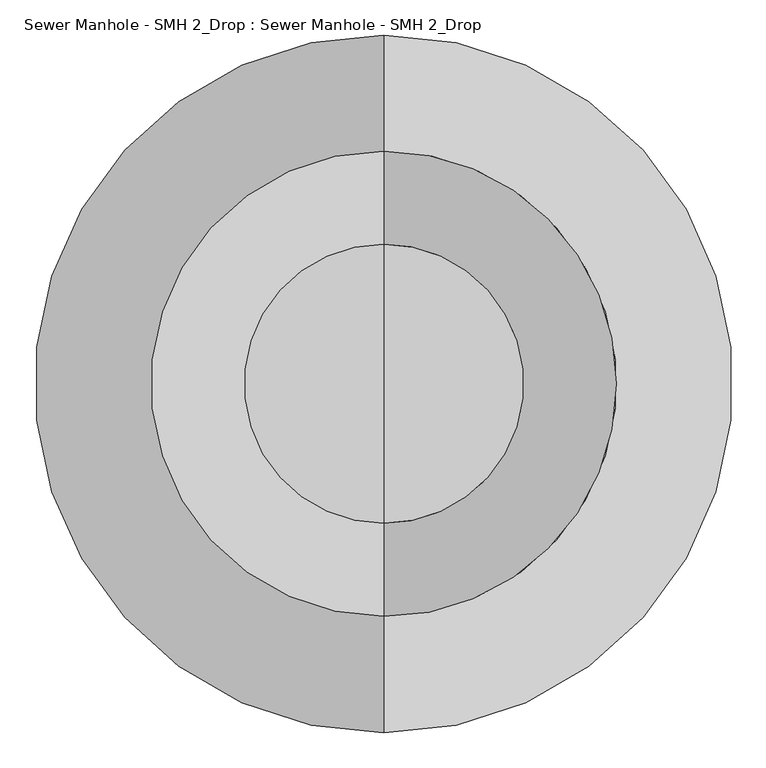
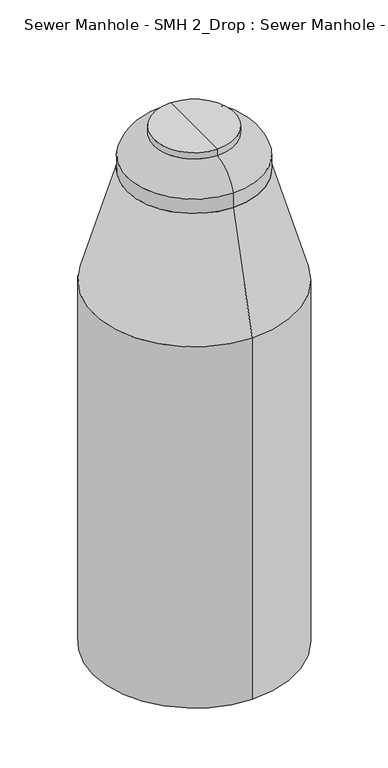
"""IFC4 building model written with IfcOpenShell, lengths in millimetres: proxy geometry, Sewer Manhole - SMH 2_Drop : Sewer Manhole - SMH 2_Drop."""

from ifc_helpers import new_model, si_unit, point, frame, origin, place, context, project, spatial, polyline, circle_curve, ellipse_curve, trimmed, source, transform, mapped, element, save
from ifc_brep_helpers import plane_surface, cylinder_surface, revolved_surface, advanced_brep


def sewer_manhole_smh_2_drop_sewer_manhole_smh_2_drop_288f05b1(model_context):
    return source(origin(), model_context, "Body", "AdvancedBrep", [
        advanced_brep(
        [(0.0, 508.0, 3771.1270774), (0.0, -508.0, 3771.1270774), (0.0, 762.0, 2885.44), (0.0, -762.0, 2885.44)],
        [
            (0, 1, circle_curve(frame((0.0, 0.0, 3771.1270774), z_axis=(0.0, 0.0, 1.0), x_axis=(0.0, 1.0, 0.0)), 508.0)),
            (1, 0, circle_curve(frame((0.0, 0.0, 3771.1270774), z_axis=(0.0, 0.0, 1.0), x_axis=(0.0, -1.0, 0.0)), 508.0)),
            (2, 3, circle_curve(frame((0.0, 0.0, 2885.44), z_axis=(0.0, 0.0, -1.0), x_axis=(0.0, -1.0, 0.0)), 762.0)),
            (3, 2, circle_curve(frame((0.0, 0.0, 2885.44), z_axis=(0.0, 0.0, -1.0), x_axis=(0.0, 1.0, 0.0)), 762.0)),
            (3, 1),
            (0, 2),
        ],
        [
            plane_surface(frame((0.0, 0.0, 3771.1270774), z_axis=(0.0, 0.0, 1.0), x_axis=(1.0, 0.0, 0.0))),
            plane_surface(frame((0.0, 0.0, 2885.44), z_axis=(0.0, 0.0, -1.0), x_axis=(1.0, 0.0, 0.0))),
            revolved_surface(polyline([(0.0, 508.00000000955947, 3771.1270774), (0.0, 762.0, 2885.44)]), (0.0, 0.0, 5542.5012323), (0.0, 0.0, -1.0)),
            revolved_surface(polyline([(0.0, -508.00000000955947, 3771.1270774), (0.0, -762.0, 2885.44)]), (0.0, 0.0, 5542.5012323), (0.0, 0.0, -1.0)),
        ],
        [
            (0, [[1, 2]]),
            (1, [[3, 4]]),
            (2, [[-4, 5, -1, 6]]),
            (3, [[-3, -6, -2, -5]]),
        ],
    ),
        advanced_brep(
        [(0.0, -508.0, 3771.1270774), (0.0, 508.0, 3771.1270774), (0.0, 0.0, 3771.1270774), (0.0, -508.0, 3886.2), (0.0, 508.0, 3886.2), (0.0, -304.8, 4064.0), (0.0, 304.8, 4064.0), (0.0, -304.8, 4114.8), (0.0, 304.8, 4114.8), (0.0, 0.0, 4114.8)],
        [
            (0, 1, circle_curve(frame((0.0, 0.0, 3771.1270774), z_axis=(0.0, 0.0, -1.0), x_axis=(0.0, 1.0, 0.0)), 508.0)),
            (1, 2),
            (2, 0),
            (1, 0, circle_curve(frame((0.0, 0.0, 3771.1270774), z_axis=(0.0, 0.0, -1.0), x_axis=(0.0, 1.0, 0.0)), 508.0)),
            (3, 4, circle_curve(frame((0.0, 0.0, 3886.2), z_axis=(0.0, 0.0, -1.0), x_axis=(0.0, 1.0, 0.0)), 508.0)),
            (4, 1),
            (0, 3),
            (4, 3, circle_curve(frame((0.0, 0.0, 3886.2), z_axis=(0.0, 0.0, -1.0), x_axis=(0.0, 1.0, 0.0)), 508.0)),
            (5, 6, circle_curve(frame((0.0, 0.0, 4064.0), z_axis=(0.0, 0.0, -1.0), x_axis=(0.0, 1.0, 0.0)), 304.8)),
            (6, 4, circle_curve(frame((0.0, 259.6539436, 3807.3902213), z_axis=(-1.0, 0.0, 0.0), x_axis=(0.0, -1.0, 0.0)), 260.550849)),
            (3, 5, circle_curve(frame((0.0, -259.6539436, 3807.3902213), z_axis=(-1.0, 0.0, 0.0), x_axis=(0.0, 1.0, 0.0)), 260.550849)),
            (6, 5, circle_curve(frame((0.0, 0.0, 4064.0), z_axis=(0.0, 0.0, -1.0), x_axis=(0.0, 1.0, 0.0)), 304.8)),
            (7, 8, circle_curve(frame((0.0, 0.0, 4114.8), z_axis=(0.0, 0.0, -1.0), x_axis=(0.0, 1.0, 0.0)), 304.8)),
            (8, 6),
            (5, 7),
            (8, 7, circle_curve(frame((0.0, 0.0, 4114.8), z_axis=(0.0, 0.0, -1.0), x_axis=(0.0, 1.0, 0.0)), 304.8)),
            (9, 8),
            (7, 9),
        ],
        [
            plane_surface(frame((0.0, 0.0, 3771.1270774), z_axis=(0.0, 0.0, -1.0), x_axis=(0.0, 1.0, 0.0))),
            cylinder_surface(frame((0.0, 0.0, 3835.4), z_axis=(0.0, 0.0, 1.0), x_axis=(0.0, 1.0, 0.0)), 508.0),
            revolved_surface(trimmed(ellipse_curve(frame((0.0, 259.6539436, 3807.3902213), z_axis=(1.0, 0.0, 0.0), x_axis=(0.0, -1.0, 0.0)), 260.550849, 260.550849), [point((0.0, 508.0, 3886.2))], [point((0.0, 304.8, 4064.0))], True, "CARTESIAN"), (0.0, 0.0, 3835.4), (0.0, 0.0, 1.0)),
            cylinder_surface(frame((0.0, 0.0, 3835.4), z_axis=(0.0, 0.0, 1.0), x_axis=(0.0, 1.0, 0.0)), 304.8),
            plane_surface(frame((0.0, 0.0, 4114.8), z_axis=(0.0, 0.0, 1.0), x_axis=(0.0, 1.0, 0.0))),
        ],
        [
            (0, [[1, 2, 3]]),
            (0, [[4, -3, -2]]),
            (1, [[5, 6, -1, 7]]),
            (1, [[8, -7, -4, -6]]),
            (2, [[9, 10, -5, 11]]),
            (2, [[12, -11, -8, -10]]),
            (3, [[13, 14, -9, 15]]),
            (3, [[16, -15, -12, -14]]),
            (4, [[17, -13, 18]]),
            (4, [[-18, -16, -17]]),
        ],
    ),
        advanced_brep(
        [(0.0, -762.0, 2885.44), (0.0, 762.0, 2885.44), (0.0, 762.0, 0.0), (0.0, -762.0, 0.0), (0.0, 0.0, 0.0), (0.0, 0.0, 2885.44)],
        [
            (0, 1, circle_curve(frame((0.0, 0.0, 2885.44), z_axis=(0.0, 0.0, -1.0), x_axis=(0.0, 1.0, 0.0)), 762.0)),
            (1, 2),
            (2, 3, circle_curve(frame((0.0, 0.0, 0.0), z_axis=(0.0, 0.0, 1.0), x_axis=(0.0, 1.0, 0.0)), 762.0)),
            (3, 0),
            (1, 0, circle_curve(frame((0.0, 0.0, 2885.44), z_axis=(0.0, 0.0, -1.0), x_axis=(0.0, 1.0, 0.0)), 762.0)),
            (3, 2, circle_curve(frame((0.0, 0.0, 0.0), z_axis=(0.0, 0.0, 1.0), x_axis=(0.0, 1.0, 0.0)), 762.0)),
            (2, 4),
            (4, 3),
            (5, 1),
            (0, 5),
        ],
        [
            cylinder_surface(frame((0.0, 0.0, 457.2), z_axis=(0.0, 0.0, 1.0), x_axis=(0.0, 1.0, 0.0)), 762.0),
            plane_surface(frame((0.0, 0.0, 0.0), z_axis=(0.0, 0.0, -1.0), x_axis=(0.0, 1.0, 0.0))),
            plane_surface(frame((0.0, 0.0, 2885.44), z_axis=(0.0, 0.0, 1.0), x_axis=(0.0, 1.0, 0.0))),
        ],
        [
            (0, [[1, 2, 3, 4]]),
            (0, [[5, -4, 6, -2]]),
            (1, [[-3, 7, 8]]),
            (1, [[-6, -8, -7]]),
            (2, [[9, -1, 10]]),
            (2, [[-10, -5, -9]]),
        ],
    ),
    ])


if __name__ == "__main__":
    model = new_model("IFC4")
    model_context = context("Model", 3, world=origin())
    ifc_project = project(units=[si_unit("LENGTHUNIT", "METRE", prefix="MILLI")], contexts=[model_context])
    site = spatial("IfcSite", under=ifc_project)
    building = spatial("IfcBuilding", under=site)
    placement = place(None, origin())
    sewer_manhole_smh_2_drop_sewer_manhole_smh_2_drop_shape = sewer_manhole_smh_2_drop_sewer_manhole_smh_2_drop_288f05b1(model_context)
    element("IfcBuildingElementProxy", 1, Name="Sewer Manhole - SMH 2_Drop : Sewer Manhole - SMH 2_Drop", ObjectType="Sewer Manhole - SMH 2_Drop : Sewer Manhole - SMH 2_Drop", at=placement, inside=building, context=model_context, shape_type="MappedRepresentation", body=[
        mapped(sewer_manhole_smh_2_drop_sewer_manhole_smh_2_drop_shape, transform((0.0, 0.0, 0.0), x_axis=(1.0, 0.0, 0.0), y_axis=(0.0, 1.0, 0.0), z_axis=(0.0, 0.0, 1.0))),
    ])
    save(model, "model.ifc")
